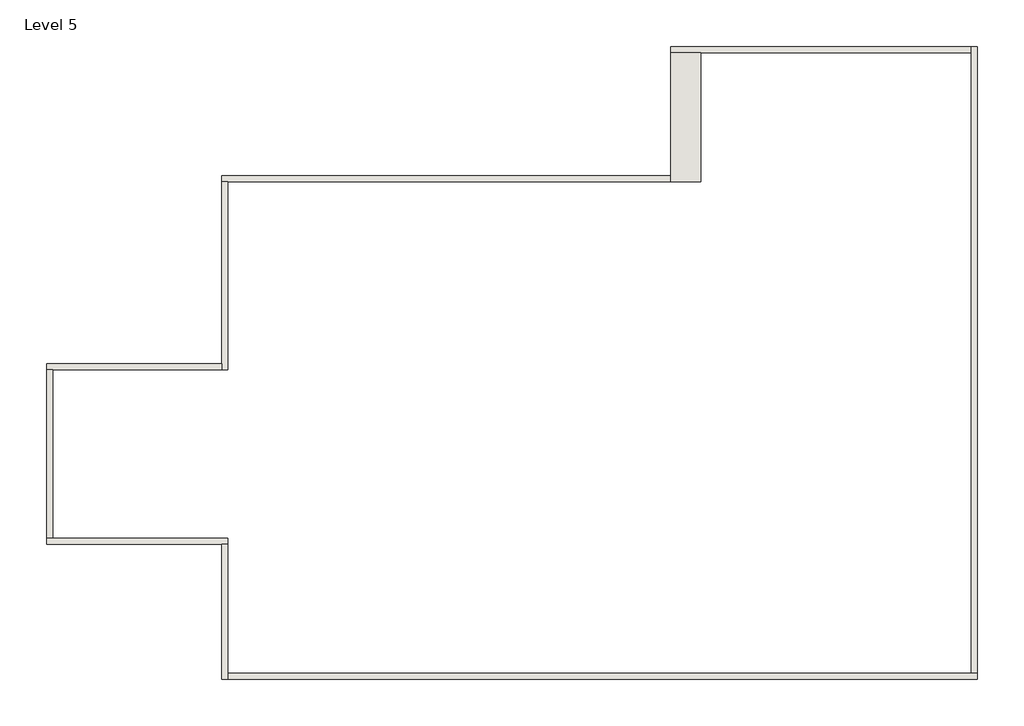
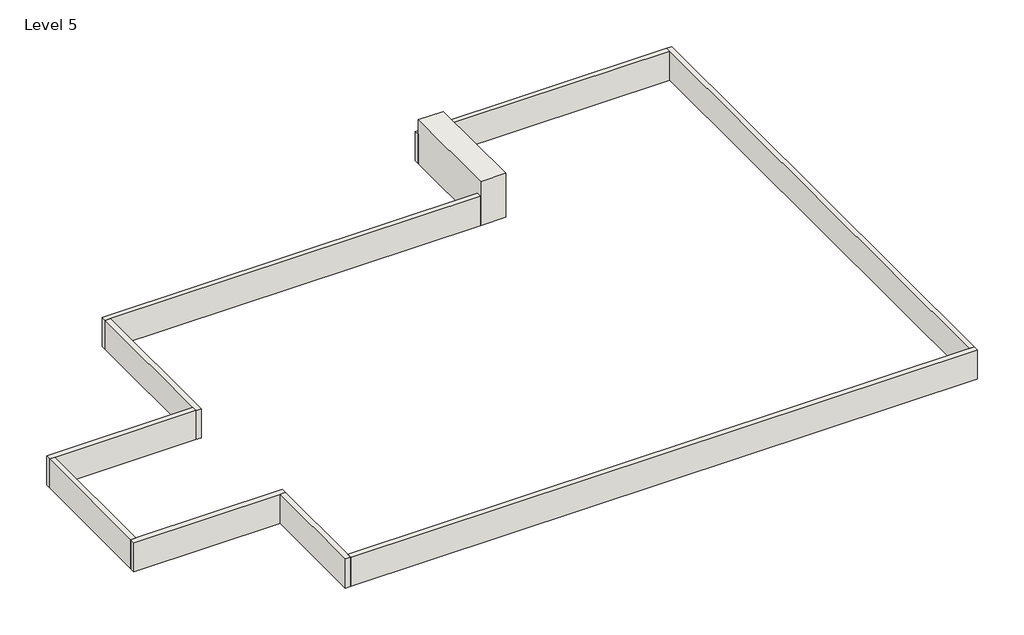
# One storey: 10 walls.
"""IFC4 building model written with IfcOpenShell, lengths in millimetres."""

from ifc_helpers import new_model, si_unit, frame, origin, place, context, project, spatial, polyline, outline, extrude, faceted_brep, element, save

model = new_model("IFC4")

# Units and contexts
model_context = context("Model", 3, world=origin())
ifc_project = project(units=[si_unit("LENGTHUNIT", "METRE", prefix="MILLI")], contexts=[model_context])

# Site, building, storey
site = spatial("IfcSite", under=ifc_project)
building = spatial("IfcBuilding", under=site)
storey = spatial("IfcBuildingStorey", under=building, Name="Level 5", Elevation=-914.4)

# Walls
placement = place(None, origin())
element("IfcWall", 1, ObjectType="foundationwall", at=placement, inside=storey, context=model_context, shape_type="Brep", body=[
    faceted_brep([(-11393.5648468, 3591.8458836, -914.4), (-8497.9648468, 3591.8458836, -914.4), (-8396.3648468, 3591.8458836, -914.4), (-8396.3648468, 3591.8458836, -304.8), (-8497.9648468, 3591.8458836, -304.8), (-11393.5648468, 3591.8458836, -304.8), (-11393.5648468, 3693.4458836, -914.4), (-11393.5648468, 3693.4458836, -304.8), (-11291.9648468, 3693.4458836, -304.8), (-8396.3648468, 3693.4458836, -304.8), (-8396.3648468, 3693.4458836, -914.4), (-11291.9648468, 3693.4458836, -914.4)], [[[0, 1, 2, 3, 4, 5]], [[6, 7, 8, 9, 10, 11]], [[2, 1, 0, 6, 11, 10]], [[5, 4, 3, 9, 8, 7]], [[3, 2, 10, 9]], [[0, 5, 7, 6]]]),
])
element("IfcWall", 2, ObjectType="foundationwall", at=placement, inside=storey, context=model_context, shape_type="Brep", body=[
    faceted_brep([(-8497.9648468, 3591.8458836, -914.4), (-8497.9648468, 1356.6458836, -914.4), (-8497.9648468, 1356.6458836, -304.8), (-8497.9648468, 3591.8458836, -304.8), (-8396.3648468, 3591.8458836, -914.4), (-8396.3648468, 3591.8458836, -304.8), (-8396.3648468, 1458.2458836, -304.8), (-8396.3648468, 1356.6458836, -304.8), (-8396.3648468, 1356.6458836, -914.4), (-8396.3648468, 1458.2458836, -914.4)], [[[0, 1, 2, 3]], [[4, 5, 6, 7, 8, 9]], [[1, 0, 4, 9, 8]], [[3, 2, 7, 6, 5]], [[0, 3, 5, 4]], [[2, 1, 8, 7]]]),
])
element("IfcWall", 3, ObjectType="foundationwall", at=placement, inside=storey, context=model_context, shape_type="Brep", body=[
    faceted_brep([(-8396.3648468, 1356.6458836, -914.4), (3998.8351532, 1356.6458836, -914.4), (3998.8351532, 1356.6458836, -304.8), (-8396.3648468, 1356.6458836, -304.8), (-8396.3648468, 1458.2458836, -914.4), (-8396.3648468, 1458.2458836, -304.8), (3897.2351532, 1458.2458836, -304.8), (3998.8351532, 1458.2458836, -304.8), (3998.8351532, 1458.2458836, -914.4), (3897.2351532, 1458.2458836, -914.4)], [[[0, 1, 2, 3]], [[4, 5, 6, 7, 8, 9]], [[1, 0, 4, 9, 8]], [[3, 2, 7, 6, 5]], [[0, 3, 5, 4]], [[2, 1, 8, 7]]]),
])
element("IfcWall", 4, ObjectType="foundationwall", at=placement, inside=storey, context=model_context, shape_type="Brep", body=[
    faceted_brep([(3998.8351532, 1458.2458836, -914.4), (3998.8351532, 11821.4458836, -914.4), (3998.8351532, 11821.4458836, -304.8), (3998.8351532, 1458.2458836, -304.8), (3897.2351532, 1458.2458836, -914.4), (3897.2351532, 1458.2458836, -304.8), (3897.2351532, 11719.8458836, -304.8), (3897.2351532, 11821.4458836, -304.8), (3897.2351532, 11821.4458836, -914.4), (3897.2351532, 11719.8458836, -914.4)], [[[0, 1, 2, 3]], [[4, 5, 6, 7, 8, 9]], [[1, 0, 4, 9, 8]], [[3, 2, 7, 6, 5]], [[0, 3, 5, 4]], [[2, 1, 8, 7]]]),
])
element("IfcWall", 5, ObjectType="foundationwall", at=placement, inside=storey, context=model_context, shape_type="Brep", body=[
    faceted_brep([(3897.2351532, 11821.4458836, -914.4), (-1074.8148468, 11821.4458836, -914.4), (-1074.8148468, 11821.4458836, -304.8), (3897.2351532, 11821.4458836, -304.8), (3897.2351532, 11719.8458836, -914.4), (3897.2351532, 11719.8458836, -304.8), (-1074.8148468, 11719.8458836, -304.8), (-1074.8148468, 11719.8458836, -914.4), (-579.5148468, 11719.8458836, -914.4)], [[[0, 1, 2, 3]], [[4, 5, 6, 7, 8]], [[1, 0, 4, 8, 7]], [[3, 2, 6, 5]], [[0, 3, 5, 4]], [[2, 1, 7, 6]]]),
])
element("IfcWall", 6, ObjectType="foundationwall", at=placement, inside=storey, context=model_context, shape_type="Brep", body=[
    faceted_brep([(-1074.8148468, 9687.8458836, -914.4), (-8497.9648468, 9687.8458836, -914.4), (-8497.9648468, 9687.8458836, -304.8), (-1074.8148468, 9687.8458836, -304.8), (-1074.8148468, 9586.2458836, -914.4), (-1074.8148468, 9586.2458836, -304.8), (-8396.3648468, 9586.2458836, -304.8), (-8497.9648468, 9586.2458836, -304.8), (-8497.9648468, 9586.2458836, -914.4), (-8396.3648468, 9586.2458836, -914.4)], [[[0, 1, 2, 3]], [[4, 5, 6, 7, 8, 9]], [[1, 0, 4, 9, 8]], [[3, 2, 7, 6, 5]], [[0, 3, 5, 4]], [[2, 1, 8, 7]]]),
])
element("IfcWall", 7, ObjectType="foundationwall", at=placement, inside=storey, context=model_context, shape_type="Brep", body=[
    faceted_brep([(-8497.9648468, 9586.2458836, -914.4), (-8497.9648468, 6580.5141758, -914.4), (-8497.9648468, 6478.9141758, -914.4), (-8497.9648468, 6478.9141758, -304.8), (-8497.9648468, 6580.5141758, -304.8), (-8497.9648468, 9586.2458836, -304.8), (-8396.3648468, 9586.2458836, -914.4), (-8396.3648468, 9586.2458836, -304.8), (-8396.3648468, 6478.9141758, -304.8), (-8396.3648468, 6478.9141758, -914.4)], [[[0, 1, 2, 3, 4, 5]], [[6, 7, 8, 9]], [[2, 1, 0, 6, 9]], [[5, 4, 3, 8, 7]], [[0, 5, 7, 6]], [[3, 2, 9, 8]]]),
])
element("IfcWall", 8, ObjectType="foundationwall", at=placement, inside=storey, context=model_context, shape_type="Brep", body=[
    faceted_brep([(-8497.9648468, 6580.5141758, -914.4), (-11393.5648468, 6580.5141758, -914.4), (-11393.5648468, 6580.5141758, -304.8), (-8497.9648468, 6580.5141758, -304.8), (-8497.9648468, 6478.9141758, -914.4), (-8497.9648468, 6478.9141758, -304.8), (-11291.9648468, 6478.9141758, -304.8), (-11393.5648468, 6478.9141758, -304.8), (-11393.5648468, 6478.9141758, -914.4), (-11291.9648468, 6478.9141758, -914.4)], [[[0, 1, 2, 3]], [[4, 5, 6, 7, 8, 9]], [[1, 0, 4, 9, 8]], [[3, 2, 7, 6, 5]], [[0, 3, 5, 4]], [[2, 1, 8, 7]]]),
])
element("IfcWall", 9, ObjectType="foundationwall", at=placement, inside=storey, context=model_context, shape_type="SweptSolid", body=[
    extrude(outline(polyline([(-11393.5648468, 3693.4458836), (-11393.5648468, 6478.9141758), (-11291.9648468, 6478.9141758), (-11291.9648468, 3693.4458836), (-11393.5648468, 3693.4458836)])), frame((0.0, 0.0, -914.4), z_axis=(0.0, 0.0, 1.0), x_axis=(1.0, 0.0, 0.0)), (0.0, 0.0, 1.0), 609.6),
])
element("IfcWall", 10, ObjectType="Exterior - Brick on CMU", at=placement, inside=storey, context=model_context, shape_type="Brep", body=[
    faceted_brep([(-1074.8148468, 11719.8458836, -914.4), (-1074.8148468, 9687.8458836, -914.4), (-1074.8148468, 9586.2458836, -914.4), (-1074.8148468, 9586.2458836, -304.8), (-1074.8148468, 9586.2458836, 0.0), (-1074.8148468, 11719.8458836, 0.0), (-1074.8148468, 11719.8458836, -304.8), (-579.5148468, 11719.8458836, -914.4), (-579.5148468, 11719.8458836, 0.0), (-579.5148468, 9586.2458836, 0.0), (-579.5148468, 9586.2458836, -914.4)], [[[0, 1, 2, 3, 4, 5, 6]], [[7, 8, 9, 10]], [[2, 1, 0, 7, 10]], [[5, 4, 9, 8]], [[0, 6, 5, 8, 7]], [[4, 3, 2, 10, 9]]]),
])

save(model, "model.ifc")

# Revit data of these elements
# Project information
#   Project Issue Date = "Issue Date"
#   Project Status = "Project Status"
#   Client Name = "Owner"
#   Project Address = "Enter address here"
#   Project Name = "Project Name"
#   Project Number = "Project Number"
# Type "foundationwall"
#   Assembly Code = "B2010"
#   Layers, outside or top first: 0' - 4" "Brick, Common" (function 1)
# Type "Exterior - Brick on CMU"
#   Assembly Code = "B2010156"
#   Layers, outside or top first: 0' - 3 5/8" "Brick, Common" (function 4); 0' - 3" "Air" (function 3); 0' - 3" "Rigid insulation" (function 3); 0' - 0" "Damp-proofing" (function 100); 0' - 7 5/8" "Concrete Masonry Units" (function 1); 0' - 1 5/8" "Metal Furring" (function 2); 0' - 0 5/8" "Gypsum Wall Board" (function 5)
# Elements 1, 2, 3, 4, 6, 7, 8, 9 (IfcWall, "foundationwall")
#   Top Offset = 0' - 0"
#   Base Offset = 0' - 0"
#   Unconnected Height = 2' - 0"
#   wall height = 2' - 0"
#   Phase Created = New Construction
#   Base Constraint = Level 5
#   Materials on its faces: "Brick, Common"
# Element 5 (IfcWall, "foundationwall")
#   Top Offset = 0' - 0"
#   Base Offset = 0' - 0"
#   Unconnected Height = 2' - 0"
#   wall height = 2' - 0"
#   Phase Created = New Construction
#   Base Constraint = Level 5
#   Materials on its faces: "Brick, Common", "Gypsum Wall Board"
# Element 10 (IfcWall, "Exterior - Brick on CMU")
#   Top Offset = 0' - 0"
#   Base Offset = 0' - 0"
#   Unconnected Height = 3' - 0"
#   wall height = 3' - 0"
#   Phase Created = New Construction
#   Base Constraint = Level 5
#   Materials on its faces: "Default Wall", "Brick, Common", "Gypsum Wall Board"
# Materials
#   "Brick, Common": class "Masonry", colour RGB 170 98 104, transparency 0, Description = "Common brick", Cost = 0
#   "Air": class "Gas", colour RGB 255 255 255, transparency 0, Description = "Air", Cost = 0
#   "Rigid insulation": class "Generic", colour RGB 127 127 127, transparency 0, Description = "Rigid foam insulation board", Cost = 0
#   "Damp-proofing": class "Generic", colour RGB 127 127 127, transparency 0, Description = "Damp-proofing", Cost = 0
#   "Concrete Masonry Units": class "Masonry", colour RGB 227 227 227, transparency 0, Description = "Concrete masonry units", Cost = 0
#   "Metal Furring": class "Metal", colour RGB 199 199 199, transparency 0, Description = "Light gauge steel furring", Cost = 0
#   "Gypsum Wall Board": class "Generic", colour RGB 127 127 127, transparency 0, Description = "Gypsum Wall Board", Cost = 0
#   "Default Wall": class "Miscellaneous", colour RGB 128 128 128, transparency 0, Cost = 0
